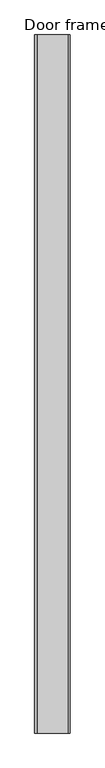
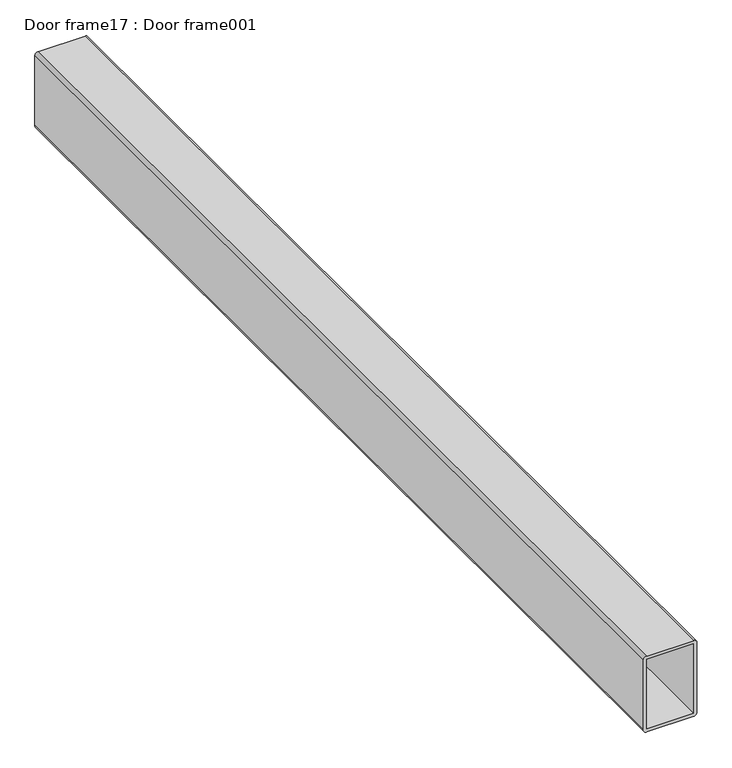
"""IFC4 building model written with IfcOpenShell, lengths in millimetres: proxy geometry, Door frame17 : Door frame001."""

import ifcopenshell
import ifcopenshell.guid

model = None  # the IFC model being written
_history = None  # IfcOwnerHistory: only IFC2X3 demands one
_inside = {}  # id of a spatial element -> (the spatial element, [elements in it])
_under = {}  # id of a project, library or spatial element -> (it, [spatial elements below it])
_declared = {}  # id of a project -> (the project, [libraries it declares])
_typed = {}  # id of a type object -> (the type object, [elements of that type])
_made_of = {}  # id of a material, layer set ... -> (it, [elements and type objects made of it])


def new_model(schema):
    """Start an empty IFC model of exactly this schema.

    Asked for "IFC4X3", IfcOpenShell would pick the latest addendum, in which some entities
    have other attributes; the version numbers below select the first issue.
    IFC2X3 requires an IfcOwnerHistory on every rooted entity: one is made here for all.
    """
    global model, _history
    if schema == "IFC4X3":
        model = ifcopenshell.file(schema_version=(4, 3, 0, 0))
    else:
        model = ifcopenshell.file(schema=schema)
    _inside.clear()
    _under.clear()
    _declared.clear()
    _typed.clear()
    _made_of.clear()
    _history = None
    if model.schema == "IFC2X3":
        org = make("IfcOrganization", Name="unknown")
        user = make(
            "IfcPersonAndOrganization",
            ThePerson=make("IfcPerson", FamilyName="unknown"),
            TheOrganization=org,
        )
        app = make(
            "IfcApplication",
            ApplicationDeveloper=org,
            Version="unknown",
            ApplicationFullName="unknown",
            ApplicationIdentifier="unknown",
        )
        _history = make(
            "IfcOwnerHistory",
            OwningUser=user,
            OwningApplication=app,
            ChangeAction="ADDED",
            CreationDate=0,
        )
    return model


def make(cls, **values):
    """One entity of the class cls with the attributes given. An attribute that is None is left unset."""
    return model.create_entity(
        cls, **{name: value for name, value in values.items() if value is not None}
    )


def rooted(cls, **values):
    """An entity with a GlobalId (a new one), such as an element, a storey or a relation."""
    return make(cls, GlobalId=ifcopenshell.guid.new(), OwnerHistory=_history, **values)


def si_unit(unit_type, name, prefix=None):
    """IfcSIUnit, for example si_unit("LENGTHUNIT", "METRE", prefix="MILLI")."""
    return make("IfcSIUnit", UnitType=unit_type, Prefix=prefix, Name=name)


def assignment(units):
    """IfcUnitAssignment: the units of a project."""
    return None if units is None else make("IfcUnitAssignment", Units=units)


def point(xyz):
    """IfcCartesianPoint."""
    return None if xyz is None else make("IfcCartesianPoint", Coordinates=xyz)


def direction(xyz):
    """IfcDirection."""
    return None if xyz is None else make("IfcDirection", DirectionRatios=xyz)


def frame(location, z_axis=None, x_axis=None):
    """IfcAxis2Placement3D, a coordinate frame: its origin and axes. An axis left out is left unset."""
    return make(
        "IfcAxis2Placement3D",
        Location=point(location),
        Axis=direction(z_axis),
        RefDirection=direction(x_axis),
    )


def frame_2d(location, x_axis=None):
    """IfcAxis2Placement2D, a coordinate frame in the plane: its origin and x axis."""
    return make(
        "IfcAxis2Placement2D", Location=point(location), RefDirection=direction(x_axis)
    )


def origin():
    """The frame at (0, 0, 0) with its axes left unset."""
    return frame((0.0, 0.0, 0.0))


def place(relative_to, where):
    """IfcLocalPlacement: puts the frame where relative to a parent placement (None: the world)."""
    return make(
        "IfcLocalPlacement", PlacementRelTo=relative_to, RelativePlacement=where
    )


def context(
    kind, dimensions, precision=None, world=None, true_north=None, identifier=None
):
    """IfcGeometricRepresentationContext, for example the 3D "Model" context."""
    return make(
        "IfcGeometricRepresentationContext",
        ContextIdentifier=identifier,
        ContextType=kind,
        CoordinateSpaceDimension=dimensions,
        Precision=precision,
        WorldCoordinateSystem=world,
        TrueNorth=true_north,
    )


def project(units=None, contexts=None):
    """IfcProject with its units and contexts."""
    return rooted(
        "IfcProject",
        Name="project",
        RepresentationContexts=contexts,
        UnitsInContext=assignment(units),
    )


def spatial(cls, under=None, at=None, **own):
    """A site, building, storey or space (cls), placed at a placement, below another one or the project."""
    s = rooted(cls, ObjectPlacement=at, **own)
    if under is not None:
        _under.setdefault(under.id(), (under, []))[1].append(s)
    return s


def polyline(points):
    """IfcPolyline through the points."""
    return make("IfcPolyline", Points=[point(p) for p in points])


def circle_curve(where, radius):
    """IfcCircle in the frame where."""
    return make("IfcCircle", Position=where, Radius=radius)


def trimmed(basis, trim1, trim2, sense, master):
    """IfcTrimmedCurve: the piece of a basis curve between two trims."""
    return make(
        "IfcTrimmedCurve",
        BasisCurve=basis,
        Trim1=trim1,
        Trim2=trim2,
        SenseAgreement=sense,
        MasterRepresentation=master,
    )


def segment(curve, same_sense, transition):
    """IfcCompositeCurveSegment."""
    return make(
        "IfcCompositeCurveSegment",
        Transition=transition,
        SameSense=same_sense,
        ParentCurve=curve,
    )


def composite_curve(segments, self_intersect=None):
    """IfcCompositeCurve: segments joined end to end."""
    return make("IfcCompositeCurve", Segments=segments, SelfIntersect=self_intersect)


def outline(outer, holes=None, kind="AREA"):
    """IfcArbitraryClosedProfileDef: a profile drawn as a closed curve; with holes, ...WithVoids."""
    if holes is None:
        return make("IfcArbitraryClosedProfileDef", ProfileType=kind, OuterCurve=outer)
    return make(
        "IfcArbitraryProfileDefWithVoids",
        ProfileType=kind,
        OuterCurve=outer,
        InnerCurves=holes,
    )


def extrude(swept, where, along, depth):
    """IfcExtrudedAreaSolid: the profile swept, set in the frame where, extruded along a direction by depth."""
    return make(
        "IfcExtrudedAreaSolid",
        SweptArea=swept,
        Position=where,
        ExtrudedDirection=direction(along),
        Depth=depth,
    )


def shape(context_of_items, identifier, shape_type, items):
    """IfcShapeRepresentation: the items that make up one representation, for example the "Body"."""
    return make(
        "IfcShapeRepresentation",
        ContextOfItems=context_of_items,
        RepresentationIdentifier=identifier,
        RepresentationType=shape_type,
        Items=items,
    )


def source(mapping_origin, context_of_items, identifier, shape_type, items):
    """IfcRepresentationMap: a shape defined once, which mapped items show again and again."""
    return make(
        "IfcRepresentationMap",
        MappingOrigin=mapping_origin,
        MappedRepresentation=shape(context_of_items, identifier, shape_type, items),
    )


def transform(
    local_origin,
    x_axis=None,
    y_axis=None,
    z_axis=None,
    scale=None,
    scale2=None,
    scale3=None,
    uniform=True,
):
    """IfcCartesianTransformationOperator3D, or its non-uniform kind. x_axis, y_axis, z_axis: its Axis1, 2, 3."""
    if uniform:
        return make(
            "IfcCartesianTransformationOperator3D",
            Axis1=direction(x_axis),
            Axis2=direction(y_axis),
            LocalOrigin=point(local_origin),
            Scale=scale,
            Axis3=direction(z_axis),
        )
    return make(
        "IfcCartesianTransformationOperator3DnonUniform",
        Axis1=direction(x_axis),
        Axis2=direction(y_axis),
        LocalOrigin=point(local_origin),
        Scale=scale,
        Axis3=direction(z_axis),
        Scale2=scale2,
        Scale3=scale3,
    )


def mapped(mapping_source, mapping_target):
    """IfcMappedItem: shows the shape of a source again, moved by a transform."""
    return make(
        "IfcMappedItem", MappingSource=mapping_source, MappingTarget=mapping_target
    )


def made_of(thing, what):
    """Note that an element or type object is made of a material, layer set ...; save() writes the relation."""
    if what is not None:
        _made_of.setdefault(what.id(), (what, []))[1].append(thing)
    return thing


def element(
    cls,
    number,
    at=None,
    inside=None,
    cuts=None,
    type_object=None,
    material=None,
    context=None,
    identifier="Body",
    shape_type=None,
    held_by="IfcProductDefinitionShape",
    body=None,
    shapes=None,
    **own,
):
    """One element of the class cls, such as IfcWall. Its Tag is "e" and its number.

    at: its placement. inside: the storey or other place that contains it. cuts: it is an
    opening in that element (IfcRelVoidsElement). A single representation is given by context,
    identifier, shape_type and body (its items); several are given by shapes. held_by: the class
    of the entity that holds the representations. save() writes the other relations.
    """
    e = rooted(cls, Tag="e%d" % number, ObjectPlacement=at, **own)
    if body is not None:
        shapes = [shape(context, identifier, shape_type, body)]
    if shapes is not None:
        e.Representation = make(held_by, Representations=shapes)
    if inside is not None:
        _inside.setdefault(inside.id(), (inside, []))[1].append(e)
    if cuts is not None:
        rooted(
            "IfcRelVoidsElement", RelatingBuildingElement=cuts, RelatedOpeningElement=e
        )
    if type_object is not None:
        _typed.setdefault(type_object.id(), (type_object, []))[1].append(e)
    return made_of(e, material)


def aggregate(whole, parts):
    """IfcRelAggregates: a whole, such as a stair, and the parts it consists of."""
    return rooted("IfcRelAggregates", RelatingObject=whole, RelatedObjects=parts)


def save(model, path):
    """Write the relations noted so far, then the file.

    IfcRelAggregates (storeys below a building ...), IfcRelContainedInSpatialStructure (elements
    in a storey), IfcRelDefinesByType, IfcRelAssociatesMaterial and IfcRelDeclares: one each for
    every whole, place, type object, material and project.
    """
    for whole, parts in _under.values():
        aggregate(whole, parts)
    for where, things in _inside.values():
        rooted(
            "IfcRelContainedInSpatialStructure",
            RelatedElements=things,
            RelatingStructure=where,
        )
    for kind, things in _typed.values():
        rooted("IfcRelDefinesByType", RelatedObjects=things, RelatingType=kind)
    for what, things in _made_of.values():
        rooted("IfcRelAssociatesMaterial", RelatedObjects=things, RelatingMaterial=what)
    for by, libraries in _declared.values():
        rooted("IfcRelDeclares", RelatingContext=by, RelatedDefinitions=libraries)
    model.write(path)


def door_frame17_door_frame001_2a17c90b(model_context):
    return source(origin(), model_context, "Body", "SweptSolid", [
        extrude(outline(composite_curve([segment(polyline([(32616.0375625, -8390.3106967), (32616.0375625, -8301.4106967)]), True, "CONTINUOUS"), segment(trimmed(circle_curve(frame_2d((32622.3875625, -8301.4106967)), 6.35), [point((32616.0375625, -8301.4106967))], [point((32622.3875625, -8295.0606967))], False, "CARTESIAN"), True, "CONTINUOUS"), segment(polyline([(32622.3875625, -8295.0606967), (32762.0875625, -8295.0606967)]), True, "CONTINUOUS"), segment(trimmed(circle_curve(frame_2d((32762.0875625, -8301.4106967)), 6.35), [point((32762.0875625, -8295.0606967))], [point((32768.4375625, -8301.4106967))], False, "CARTESIAN"), True, "CONTINUOUS"), segment(polyline([(32768.4375625, -8301.4106967), (32768.4375625, -8390.3106967)]), True, "CONTINUOUS"), segment(trimmed(circle_curve(frame_2d((32762.0875625, -8390.3106967)), 6.35), [point((32768.4375625, -8390.3106967))], [point((32762.0875625, -8396.6606967))], False, "CARTESIAN"), True, "CONTINUOUS"), segment(polyline([(32762.0875625, -8396.6606967), (32622.3875625, -8396.6606967)]), True, "CONTINUOUS"), segment(trimmed(circle_curve(frame_2d((32622.3875625, -8390.3106967)), 6.35), [point((32622.3875625, -8396.6606967))], [point((32616.0375625, -8390.3106967))], False, "CARTESIAN"), True, "CONTINUOUS")], self_intersect=False), holes=[polyline([(32761.9375625, -8301.5606967), (32622.5375625, -8301.5606967), (32622.5375625, -8390.1606967), (32761.9375625, -8390.1606967), (32761.9375625, -8301.5606967)])]), frame((0.0, 4540.4513244, 0.0), z_axis=(0.0, 1.0, 0.0), x_axis=(0.0, 0.0, 1.0)), (0.0, 0.0, 1.0), 2000.0),
    ])


if __name__ == "__main__":
    model = new_model("IFC4")
    model_context = context("Model", 3, world=origin())
    ifc_project = project(units=[si_unit("LENGTHUNIT", "METRE", prefix="MILLI")], contexts=[model_context])
    site = spatial("IfcSite", under=ifc_project)
    building = spatial("IfcBuilding", under=site)
    placement = place(None, origin())
    door_frame17_door_frame001_shape = door_frame17_door_frame001_2a17c90b(model_context)
    element("IfcBuildingElementProxy", 1, Name="Door frame17 : Door frame001", ObjectType="Door frame17 : Door frame001", at=placement, inside=building, context=model_context, shape_type="MappedRepresentation", body=[
        mapped(door_frame17_door_frame001_shape, transform((0.0, 0.0, 0.0), x_axis=(1.0, 0.0, 0.0), y_axis=(0.0, 1.0, 0.0), z_axis=(0.0, 0.0, 1.0))),
    ])
    save(model, "model.ifc")

# Revit data of these elements
# Type "Door frame17 : Door frame001"
#   NameOverride = "Door frame001"
# Element 1 (IfcBuildingElementProxy, "Door frame17 : Door frame001")
#   Materials on its faces: "DOOR FRAME: TUBE STEEL PROFILE - METALIZED, PRIMED & PAINTED (COLOR PER ARCHITECT)"
# Materials
#   "DOOR FRAME: TUBE STEEL PROFILE - METALIZED, PRIMED & PAINTED (COLOR PER ARCHITECT)": class "Unassigned", colour RGB 128 128 128, transparency 0, Cost = 0
